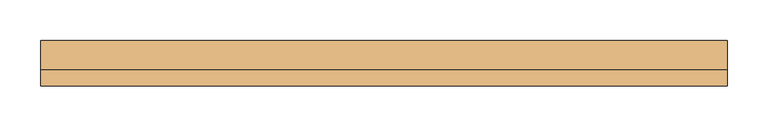
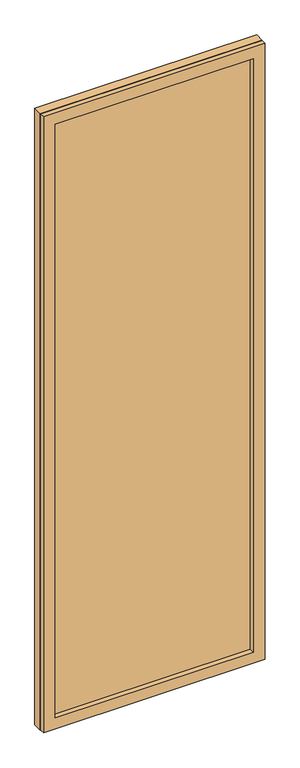
"""IFC4 building model written with IfcOpenShell, lengths in millimetres: door geometry, Anta Singola SENZA MANIGLIA(1) : Anta Singola SENZA MANIGLIA(1)."""

import ifcopenshell
import ifcopenshell.guid

model = None  # the IFC model being written
_history = None  # IfcOwnerHistory: only IFC2X3 demands one
_inside = {}  # id of a spatial element -> (the spatial element, [elements in it])
_under = {}  # id of a project, library or spatial element -> (it, [spatial elements below it])
_declared = {}  # id of a project -> (the project, [libraries it declares])
_typed = {}  # id of a type object -> (the type object, [elements of that type])
_made_of = {}  # id of a material, layer set ... -> (it, [elements and type objects made of it])


def new_model(schema):
    """Start an empty IFC model of exactly this schema.

    Asked for "IFC4X3", IfcOpenShell would pick the latest addendum, in which some entities
    have other attributes; the version numbers below select the first issue.
    IFC2X3 requires an IfcOwnerHistory on every rooted entity: one is made here for all.
    """
    global model, _history
    if schema == "IFC4X3":
        model = ifcopenshell.file(schema_version=(4, 3, 0, 0))
    else:
        model = ifcopenshell.file(schema=schema)
    _inside.clear()
    _under.clear()
    _declared.clear()
    _typed.clear()
    _made_of.clear()
    _history = None
    if model.schema == "IFC2X3":
        org = make("IfcOrganization", Name="unknown")
        user = make(
            "IfcPersonAndOrganization",
            ThePerson=make("IfcPerson", FamilyName="unknown"),
            TheOrganization=org,
        )
        app = make(
            "IfcApplication",
            ApplicationDeveloper=org,
            Version="unknown",
            ApplicationFullName="unknown",
            ApplicationIdentifier="unknown",
        )
        _history = make(
            "IfcOwnerHistory",
            OwningUser=user,
            OwningApplication=app,
            ChangeAction="ADDED",
            CreationDate=0,
        )
    return model


def make(cls, **values):
    """One entity of the class cls with the attributes given. An attribute that is None is left unset."""
    return model.create_entity(
        cls, **{name: value for name, value in values.items() if value is not None}
    )


def rooted(cls, **values):
    """An entity with a GlobalId (a new one), such as an element, a storey or a relation."""
    return make(cls, GlobalId=ifcopenshell.guid.new(), OwnerHistory=_history, **values)


def si_unit(unit_type, name, prefix=None):
    """IfcSIUnit, for example si_unit("LENGTHUNIT", "METRE", prefix="MILLI")."""
    return make("IfcSIUnit", UnitType=unit_type, Prefix=prefix, Name=name)


def assignment(units):
    """IfcUnitAssignment: the units of a project."""
    return None if units is None else make("IfcUnitAssignment", Units=units)


def point(xyz):
    """IfcCartesianPoint."""
    return None if xyz is None else make("IfcCartesianPoint", Coordinates=xyz)


def direction(xyz):
    """IfcDirection."""
    return None if xyz is None else make("IfcDirection", DirectionRatios=xyz)


def frame(location, z_axis=None, x_axis=None):
    """IfcAxis2Placement3D, a coordinate frame: its origin and axes. An axis left out is left unset."""
    return make(
        "IfcAxis2Placement3D",
        Location=point(location),
        Axis=direction(z_axis),
        RefDirection=direction(x_axis),
    )


def origin():
    """The frame at (0, 0, 0) with its axes left unset."""
    return frame((0.0, 0.0, 0.0))


def place(relative_to, where):
    """IfcLocalPlacement: puts the frame where relative to a parent placement (None: the world)."""
    return make(
        "IfcLocalPlacement", PlacementRelTo=relative_to, RelativePlacement=where
    )


def context(
    kind, dimensions, precision=None, world=None, true_north=None, identifier=None
):
    """IfcGeometricRepresentationContext, for example the 3D "Model" context."""
    return make(
        "IfcGeometricRepresentationContext",
        ContextIdentifier=identifier,
        ContextType=kind,
        CoordinateSpaceDimension=dimensions,
        Precision=precision,
        WorldCoordinateSystem=world,
        TrueNorth=true_north,
    )


def project(units=None, contexts=None):
    """IfcProject with its units and contexts."""
    return rooted(
        "IfcProject",
        Name="project",
        RepresentationContexts=contexts,
        UnitsInContext=assignment(units),
    )


def spatial(cls, under=None, at=None, **own):
    """A site, building, storey or space (cls), placed at a placement, below another one or the project."""
    s = rooted(cls, ObjectPlacement=at, **own)
    if under is not None:
        _under.setdefault(under.id(), (under, []))[1].append(s)
    return s


def polyline(points):
    """IfcPolyline through the points."""
    return make("IfcPolyline", Points=[point(p) for p in points])


def outline(outer, holes=None, kind="AREA"):
    """IfcArbitraryClosedProfileDef: a profile drawn as a closed curve; with holes, ...WithVoids."""
    if holes is None:
        return make("IfcArbitraryClosedProfileDef", ProfileType=kind, OuterCurve=outer)
    return make(
        "IfcArbitraryProfileDefWithVoids",
        ProfileType=kind,
        OuterCurve=outer,
        InnerCurves=holes,
    )


def extrude(swept, where, along, depth):
    """IfcExtrudedAreaSolid: the profile swept, set in the frame where, extruded along a direction by depth."""
    return make(
        "IfcExtrudedAreaSolid",
        SweptArea=swept,
        Position=where,
        ExtrudedDirection=direction(along),
        Depth=depth,
    )


def shape(context_of_items, identifier, shape_type, items):
    """IfcShapeRepresentation: the items that make up one representation, for example the "Body"."""
    return make(
        "IfcShapeRepresentation",
        ContextOfItems=context_of_items,
        RepresentationIdentifier=identifier,
        RepresentationType=shape_type,
        Items=items,
    )


def source(mapping_origin, context_of_items, identifier, shape_type, items):
    """IfcRepresentationMap: a shape defined once, which mapped items show again and again."""
    return make(
        "IfcRepresentationMap",
        MappingOrigin=mapping_origin,
        MappedRepresentation=shape(context_of_items, identifier, shape_type, items),
    )


def transform(
    local_origin,
    x_axis=None,
    y_axis=None,
    z_axis=None,
    scale=None,
    scale2=None,
    scale3=None,
    uniform=True,
):
    """IfcCartesianTransformationOperator3D, or its non-uniform kind. x_axis, y_axis, z_axis: its Axis1, 2, 3."""
    if uniform:
        return make(
            "IfcCartesianTransformationOperator3D",
            Axis1=direction(x_axis),
            Axis2=direction(y_axis),
            LocalOrigin=point(local_origin),
            Scale=scale,
            Axis3=direction(z_axis),
        )
    return make(
        "IfcCartesianTransformationOperator3DnonUniform",
        Axis1=direction(x_axis),
        Axis2=direction(y_axis),
        LocalOrigin=point(local_origin),
        Scale=scale,
        Axis3=direction(z_axis),
        Scale2=scale2,
        Scale3=scale3,
    )


def mapped(mapping_source, mapping_target):
    """IfcMappedItem: shows the shape of a source again, moved by a transform."""
    return make(
        "IfcMappedItem", MappingSource=mapping_source, MappingTarget=mapping_target
    )


def made_of(thing, what):
    """Note that an element or type object is made of a material, layer set ...; save() writes the relation."""
    if what is not None:
        _made_of.setdefault(what.id(), (what, []))[1].append(thing)
    return thing


def element(
    cls,
    number,
    at=None,
    inside=None,
    cuts=None,
    type_object=None,
    material=None,
    context=None,
    identifier="Body",
    shape_type=None,
    held_by="IfcProductDefinitionShape",
    body=None,
    shapes=None,
    **own,
):
    """One element of the class cls, such as IfcWall. Its Tag is "e" and its number.

    at: its placement. inside: the storey or other place that contains it. cuts: it is an
    opening in that element (IfcRelVoidsElement). A single representation is given by context,
    identifier, shape_type and body (its items); several are given by shapes. held_by: the class
    of the entity that holds the representations. save() writes the other relations.
    """
    e = rooted(cls, Tag="e%d" % number, ObjectPlacement=at, **own)
    if body is not None:
        shapes = [shape(context, identifier, shape_type, body)]
    if shapes is not None:
        e.Representation = make(held_by, Representations=shapes)
    if inside is not None:
        _inside.setdefault(inside.id(), (inside, []))[1].append(e)
    if cuts is not None:
        rooted(
            "IfcRelVoidsElement", RelatingBuildingElement=cuts, RelatedOpeningElement=e
        )
    if type_object is not None:
        _typed.setdefault(type_object.id(), (type_object, []))[1].append(e)
    return made_of(e, material)


def aggregate(whole, parts):
    """IfcRelAggregates: a whole, such as a stair, and the parts it consists of."""
    return rooted("IfcRelAggregates", RelatingObject=whole, RelatedObjects=parts)


def save(model, path):
    """Write the relations noted so far, then the file.

    IfcRelAggregates (storeys below a building ...), IfcRelContainedInSpatialStructure (elements
    in a storey), IfcRelDefinesByType, IfcRelAssociatesMaterial and IfcRelDeclares: one each for
    every whole, place, type object, material and project.
    """
    for whole, parts in _under.values():
        aggregate(whole, parts)
    for where, things in _inside.values():
        rooted(
            "IfcRelContainedInSpatialStructure",
            RelatedElements=things,
            RelatingStructure=where,
        )
    for kind, things in _typed.values():
        rooted("IfcRelDefinesByType", RelatedObjects=things, RelatingType=kind)
    for what, things in _made_of.values():
        rooted("IfcRelAssociatesMaterial", RelatedObjects=things, RelatingMaterial=what)
    for by, libraries in _declared.values():
        rooted("IfcRelDeclares", RelatingContext=by, RelatedDefinitions=libraries)
    model.write(path)


def door_5512adb9(model_context):
    return source(origin(), model_context, "Body", "SweptSolid", [
        extrude(outline(polyline([(422.5, -18.0), (-422.5, -18.0), (-422.5, 18.0), (422.5, 18.0), (422.5, -18.0)])), frame((0.0, 0.0, -3.1739529), z_axis=(0.0, 0.0, 1.0), x_axis=(1.0, 0.0, 0.0)), (0.0, 0.0, 1.0), 2478.1739529),
        extrude(outline(polyline([(2474.5625024, 422.0625024), (2474.5625024, -422.0625024), (-2.7364552, -422.0625024), (-2.7364552, 422.0625024), (2474.5625024, 422.0625024)]), holes=[polyline([(2429.5625024, -377.0625024), (2429.5625024, 377.0625024), (42.2635448, 377.0625024), (42.2635448, -377.0625024), (2429.5625024, -377.0625024)])]), frame((0.0, -38.0, 0.0), z_axis=(0.0, 1.0, 0.0), x_axis=(0.0, 0.0, 1.0)), (0.0, 0.0, 1.0), 20.0),
    ])


if __name__ == "__main__":
    model = new_model("IFC4")
    model_context = context("Model", 3, world=origin())
    ifc_project = project(units=[si_unit("LENGTHUNIT", "METRE", prefix="MILLI")], contexts=[model_context])
    site = spatial("IfcSite", under=ifc_project)
    building = spatial("IfcBuilding", under=site)
    placement = place(None, origin())
    door_shape = door_5512adb9(model_context)
    element("IfcDoor", 1, ObjectType="Anta Singola SENZA MANIGLIA(1) : Anta Singola SENZA MANIGLIA(1)", at=placement, inside=building, context=model_context, shape_type="MappedRepresentation", body=[
        mapped(door_shape, transform((0.0, 0.0, 0.0), x_axis=(1.0, 0.0, 0.0), y_axis=(0.0, 1.0, 0.0), z_axis=(0.0, 0.0, 1.0))),
    ])
    save(model, "model.ifc")

# Revit data of these elements
# Type "Anta Singola SENZA MANIGLIA(1) : Anta Singola SENZA MANIGLIA(1)"
#   Type Mark = "15"
#   Construction Type = "Scorrimenti"
#   Construction Type Id = "opn-d42"
#   Analytic Construction = "Telaio in metallo con vetro singolo trasparente"
#   Sp = 0.036 m
#   Thermal Resistance (R) = 0.152486 (m²·K)/W
#   Heat Transfer Coefficient (U) = 6.5580 W/(m²·K)
#   L cornice = 0.045 m
#   Quadro = Default - Vetro
#   Maniglia = none
#   Visual Light Transmittance = 0
#   Solar Heat Gain Coefficient = 0
#   Manufacturer = ""
#   Function = (empty or 0)
# Element 1 (IfcDoor, "Anta Singola SENZA MANIGLIA(1) : Anta Singola SENZA MANIGLIA(1)")
#   Materials on its faces: "Maniglia", "Default - Vetro"
# Materials
#   "Default - Vetro": class "Vetro", colour RGB 208 208 208, transparency 0.7, Cost = 0
#   "Maniglia": class "Varie", colour RGB 219 219 219, transparency 0
